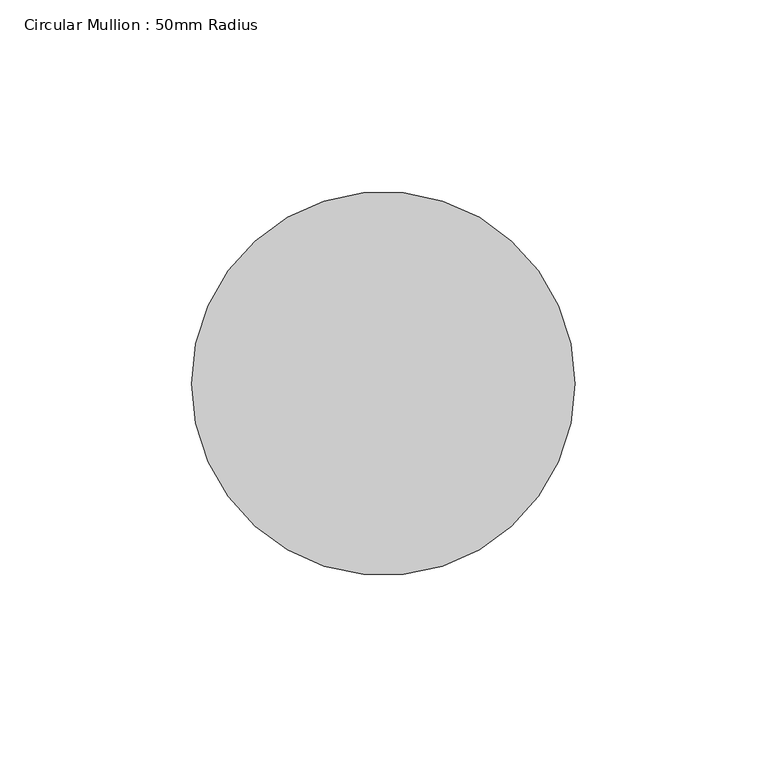
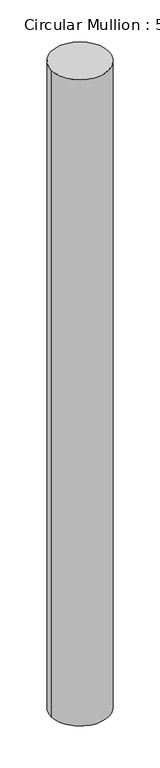
"""IFC4 building model written with IfcOpenShell, lengths in millimetres: member geometry, Circular Mullion : 50mm Radius."""

import ifcopenshell
import ifcopenshell.guid

model = None  # the IFC model being written
_history = None  # IfcOwnerHistory: only IFC2X3 demands one
_inside = {}  # id of a spatial element -> (the spatial element, [elements in it])
_under = {}  # id of a project, library or spatial element -> (it, [spatial elements below it])
_declared = {}  # id of a project -> (the project, [libraries it declares])
_typed = {}  # id of a type object -> (the type object, [elements of that type])
_made_of = {}  # id of a material, layer set ... -> (it, [elements and type objects made of it])


def new_model(schema):
    """Start an empty IFC model of exactly this schema.

    Asked for "IFC4X3", IfcOpenShell would pick the latest addendum, in which some entities
    have other attributes; the version numbers below select the first issue.
    IFC2X3 requires an IfcOwnerHistory on every rooted entity: one is made here for all.
    """
    global model, _history
    if schema == "IFC4X3":
        model = ifcopenshell.file(schema_version=(4, 3, 0, 0))
    else:
        model = ifcopenshell.file(schema=schema)
    _inside.clear()
    _under.clear()
    _declared.clear()
    _typed.clear()
    _made_of.clear()
    _history = None
    if model.schema == "IFC2X3":
        org = make("IfcOrganization", Name="unknown")
        user = make(
            "IfcPersonAndOrganization",
            ThePerson=make("IfcPerson", FamilyName="unknown"),
            TheOrganization=org,
        )
        app = make(
            "IfcApplication",
            ApplicationDeveloper=org,
            Version="unknown",
            ApplicationFullName="unknown",
            ApplicationIdentifier="unknown",
        )
        _history = make(
            "IfcOwnerHistory",
            OwningUser=user,
            OwningApplication=app,
            ChangeAction="ADDED",
            CreationDate=0,
        )
    return model


def make(cls, **values):
    """One entity of the class cls with the attributes given. An attribute that is None is left unset."""
    return model.create_entity(
        cls, **{name: value for name, value in values.items() if value is not None}
    )


def rooted(cls, **values):
    """An entity with a GlobalId (a new one), such as an element, a storey or a relation."""
    return make(cls, GlobalId=ifcopenshell.guid.new(), OwnerHistory=_history, **values)


def si_unit(unit_type, name, prefix=None):
    """IfcSIUnit, for example si_unit("LENGTHUNIT", "METRE", prefix="MILLI")."""
    return make("IfcSIUnit", UnitType=unit_type, Prefix=prefix, Name=name)


def assignment(units):
    """IfcUnitAssignment: the units of a project."""
    return None if units is None else make("IfcUnitAssignment", Units=units)


def point(xyz):
    """IfcCartesianPoint."""
    return None if xyz is None else make("IfcCartesianPoint", Coordinates=xyz)


def direction(xyz):
    """IfcDirection."""
    return None if xyz is None else make("IfcDirection", DirectionRatios=xyz)


def frame(location, z_axis=None, x_axis=None):
    """IfcAxis2Placement3D, a coordinate frame: its origin and axes. An axis left out is left unset."""
    return make(
        "IfcAxis2Placement3D",
        Location=point(location),
        Axis=direction(z_axis),
        RefDirection=direction(x_axis),
    )


def frame_2d(location, x_axis=None):
    """IfcAxis2Placement2D, a coordinate frame in the plane: its origin and x axis."""
    return make(
        "IfcAxis2Placement2D", Location=point(location), RefDirection=direction(x_axis)
    )


def origin():
    """The frame at (0, 0, 0) with its axes left unset."""
    return frame((0.0, 0.0, 0.0))


def origin_2d():
    """The frame at (0, 0) in the plane with its x axis left unset."""
    return frame_2d((0.0, 0.0))


def place(relative_to, where):
    """IfcLocalPlacement: puts the frame where relative to a parent placement (None: the world)."""
    return make(
        "IfcLocalPlacement", PlacementRelTo=relative_to, RelativePlacement=where
    )


def context(
    kind, dimensions, precision=None, world=None, true_north=None, identifier=None
):
    """IfcGeometricRepresentationContext, for example the 3D "Model" context."""
    return make(
        "IfcGeometricRepresentationContext",
        ContextIdentifier=identifier,
        ContextType=kind,
        CoordinateSpaceDimension=dimensions,
        Precision=precision,
        WorldCoordinateSystem=world,
        TrueNorth=true_north,
    )


def project(units=None, contexts=None):
    """IfcProject with its units and contexts."""
    return rooted(
        "IfcProject",
        Name="project",
        RepresentationContexts=contexts,
        UnitsInContext=assignment(units),
    )


def spatial(cls, under=None, at=None, **own):
    """A site, building, storey or space (cls), placed at a placement, below another one or the project."""
    s = rooted(cls, ObjectPlacement=at, **own)
    if under is not None:
        _under.setdefault(under.id(), (under, []))[1].append(s)
    return s


def circle_curve(where, radius):
    """IfcCircle in the frame where."""
    return make("IfcCircle", Position=where, Radius=radius)


def trimmed(basis, trim1, trim2, sense, master):
    """IfcTrimmedCurve: the piece of a basis curve between two trims."""
    return make(
        "IfcTrimmedCurve",
        BasisCurve=basis,
        Trim1=trim1,
        Trim2=trim2,
        SenseAgreement=sense,
        MasterRepresentation=master,
    )


def segment(curve, same_sense, transition):
    """IfcCompositeCurveSegment."""
    return make(
        "IfcCompositeCurveSegment",
        Transition=transition,
        SameSense=same_sense,
        ParentCurve=curve,
    )


def composite_curve(segments, self_intersect=None):
    """IfcCompositeCurve: segments joined end to end."""
    return make("IfcCompositeCurve", Segments=segments, SelfIntersect=self_intersect)


def outline(outer, holes=None, kind="AREA"):
    """IfcArbitraryClosedProfileDef: a profile drawn as a closed curve; with holes, ...WithVoids."""
    if holes is None:
        return make("IfcArbitraryClosedProfileDef", ProfileType=kind, OuterCurve=outer)
    return make(
        "IfcArbitraryProfileDefWithVoids",
        ProfileType=kind,
        OuterCurve=outer,
        InnerCurves=holes,
    )


def extrude(swept, where, along, depth):
    """IfcExtrudedAreaSolid: the profile swept, set in the frame where, extruded along a direction by depth."""
    return make(
        "IfcExtrudedAreaSolid",
        SweptArea=swept,
        Position=where,
        ExtrudedDirection=direction(along),
        Depth=depth,
    )


def shape(context_of_items, identifier, shape_type, items):
    """IfcShapeRepresentation: the items that make up one representation, for example the "Body"."""
    return make(
        "IfcShapeRepresentation",
        ContextOfItems=context_of_items,
        RepresentationIdentifier=identifier,
        RepresentationType=shape_type,
        Items=items,
    )


def source(mapping_origin, context_of_items, identifier, shape_type, items):
    """IfcRepresentationMap: a shape defined once, which mapped items show again and again."""
    return make(
        "IfcRepresentationMap",
        MappingOrigin=mapping_origin,
        MappedRepresentation=shape(context_of_items, identifier, shape_type, items),
    )


def transform(
    local_origin,
    x_axis=None,
    y_axis=None,
    z_axis=None,
    scale=None,
    scale2=None,
    scale3=None,
    uniform=True,
):
    """IfcCartesianTransformationOperator3D, or its non-uniform kind. x_axis, y_axis, z_axis: its Axis1, 2, 3."""
    if uniform:
        return make(
            "IfcCartesianTransformationOperator3D",
            Axis1=direction(x_axis),
            Axis2=direction(y_axis),
            LocalOrigin=point(local_origin),
            Scale=scale,
            Axis3=direction(z_axis),
        )
    return make(
        "IfcCartesianTransformationOperator3DnonUniform",
        Axis1=direction(x_axis),
        Axis2=direction(y_axis),
        LocalOrigin=point(local_origin),
        Scale=scale,
        Axis3=direction(z_axis),
        Scale2=scale2,
        Scale3=scale3,
    )


def mapped(mapping_source, mapping_target):
    """IfcMappedItem: shows the shape of a source again, moved by a transform."""
    return make(
        "IfcMappedItem", MappingSource=mapping_source, MappingTarget=mapping_target
    )


def made_of(thing, what):
    """Note that an element or type object is made of a material, layer set ...; save() writes the relation."""
    if what is not None:
        _made_of.setdefault(what.id(), (what, []))[1].append(thing)
    return thing


def element(
    cls,
    number,
    at=None,
    inside=None,
    cuts=None,
    type_object=None,
    material=None,
    context=None,
    identifier="Body",
    shape_type=None,
    held_by="IfcProductDefinitionShape",
    body=None,
    shapes=None,
    **own,
):
    """One element of the class cls, such as IfcWall. Its Tag is "e" and its number.

    at: its placement. inside: the storey or other place that contains it. cuts: it is an
    opening in that element (IfcRelVoidsElement). A single representation is given by context,
    identifier, shape_type and body (its items); several are given by shapes. held_by: the class
    of the entity that holds the representations. save() writes the other relations.
    """
    e = rooted(cls, Tag="e%d" % number, ObjectPlacement=at, **own)
    if body is not None:
        shapes = [shape(context, identifier, shape_type, body)]
    if shapes is not None:
        e.Representation = make(held_by, Representations=shapes)
    if inside is not None:
        _inside.setdefault(inside.id(), (inside, []))[1].append(e)
    if cuts is not None:
        rooted(
            "IfcRelVoidsElement", RelatingBuildingElement=cuts, RelatedOpeningElement=e
        )
    if type_object is not None:
        _typed.setdefault(type_object.id(), (type_object, []))[1].append(e)
    return made_of(e, material)


def aggregate(whole, parts):
    """IfcRelAggregates: a whole, such as a stair, and the parts it consists of."""
    return rooted("IfcRelAggregates", RelatingObject=whole, RelatedObjects=parts)


def save(model, path):
    """Write the relations noted so far, then the file.

    IfcRelAggregates (storeys below a building ...), IfcRelContainedInSpatialStructure (elements
    in a storey), IfcRelDefinesByType, IfcRelAssociatesMaterial and IfcRelDeclares: one each for
    every whole, place, type object, material and project.
    """
    for whole, parts in _under.values():
        aggregate(whole, parts)
    for where, things in _inside.values():
        rooted(
            "IfcRelContainedInSpatialStructure",
            RelatedElements=things,
            RelatingStructure=where,
        )
    for kind, things in _typed.values():
        rooted("IfcRelDefinesByType", RelatedObjects=things, RelatingType=kind)
    for what, things in _made_of.values():
        rooted("IfcRelAssociatesMaterial", RelatedObjects=things, RelatingMaterial=what)
    for by, libraries in _declared.values():
        rooted("IfcRelDeclares", RelatingContext=by, RelatedDefinitions=libraries)
    model.write(path)


def circular_mullion_50mm_radius_6fe602bb(model_context):
    return source(origin(), model_context, "Body", "SweptSolid", [
        extrude(outline(composite_curve([segment(trimmed(circle_curve(origin_2d(), 50.0), [point((50.0, 0.0))], [point((-50.0, 0.0))], False, "CARTESIAN"), True, "CONTINUOUS"), segment(trimmed(circle_curve(origin_2d(), 50.0), [point((-50.0, 0.0))], [point((50.0, 0.0))], False, "CARTESIAN"), True, "CONTINUOUS")], self_intersect=False)), frame((0.0, 0.0, -1191.1471387), z_axis=(0.0, 0.0, 1.0), x_axis=(1.0, 0.0, 0.0)), (0.0, 0.0, 1.0), 1191.1471387),
    ])


if __name__ == "__main__":
    model = new_model("IFC4")
    model_context = context("Model", 3, world=origin())
    ifc_project = project(units=[si_unit("LENGTHUNIT", "METRE", prefix="MILLI")], contexts=[model_context])
    site = spatial("IfcSite", under=ifc_project)
    building = spatial("IfcBuilding", under=site)
    placement = place(None, origin())
    circular_mullion_50mm_radius_shape = circular_mullion_50mm_radius_6fe602bb(model_context)
    element("IfcMember", 1, ObjectType="Circular Mullion : 50mm Radius", at=placement, inside=building, context=model_context, shape_type="MappedRepresentation", body=[
        mapped(circular_mullion_50mm_radius_shape, transform((0.0, 0.0, 0.0), x_axis=(1.0, 0.0, 0.0), y_axis=(0.0, 1.0, 0.0), z_axis=(0.0, 0.0, 1.0))),
    ])
    save(model, "model.ifc")

# Revit data of these elements
# Type "Circular Mullion : 50mm Radius"
#   built-in parameter 1007350 = 0.164042 (stored number, unit not read)
# Element 1 (IfcMember, "Circular Mullion : 50mm Radius")
#   Materials on its faces: "Aluminium"
# Materials
#   "Aluminium": class "Metal", colour RGB 247 247 247, transparency 0, Description = "Aluminium 6061", Cost = 0
